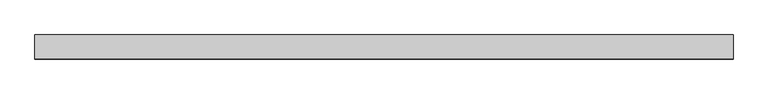
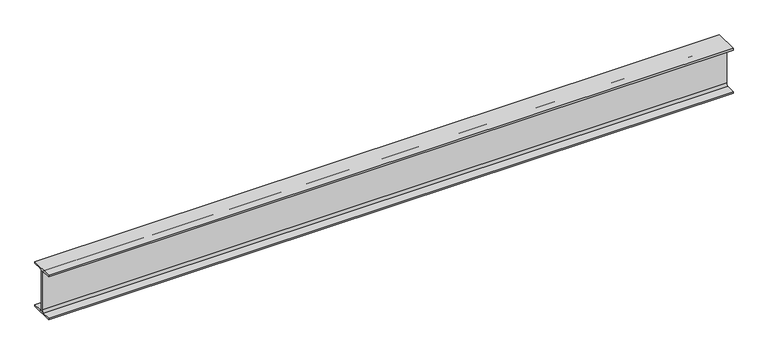
"""IFC4 building model written with IfcOpenShell, lengths in millimetres: beam geometry, 0912_Steel Framing_H-KSD3502 : H_SB_ASB_H-250x125x6x9."""

import ifcopenshell
import ifcopenshell.guid

model = None  # the IFC model being written
_history = None  # IfcOwnerHistory: only IFC2X3 demands one
_inside = {}  # id of a spatial element -> (the spatial element, [elements in it])
_under = {}  # id of a project, library or spatial element -> (it, [spatial elements below it])
_declared = {}  # id of a project -> (the project, [libraries it declares])
_typed = {}  # id of a type object -> (the type object, [elements of that type])
_made_of = {}  # id of a material, layer set ... -> (it, [elements and type objects made of it])


def new_model(schema):
    """Start an empty IFC model of exactly this schema.

    Asked for "IFC4X3", IfcOpenShell would pick the latest addendum, in which some entities
    have other attributes; the version numbers below select the first issue.
    IFC2X3 requires an IfcOwnerHistory on every rooted entity: one is made here for all.
    """
    global model, _history
    if schema == "IFC4X3":
        model = ifcopenshell.file(schema_version=(4, 3, 0, 0))
    else:
        model = ifcopenshell.file(schema=schema)
    _inside.clear()
    _under.clear()
    _declared.clear()
    _typed.clear()
    _made_of.clear()
    _history = None
    if model.schema == "IFC2X3":
        org = make("IfcOrganization", Name="unknown")
        user = make(
            "IfcPersonAndOrganization",
            ThePerson=make("IfcPerson", FamilyName="unknown"),
            TheOrganization=org,
        )
        app = make(
            "IfcApplication",
            ApplicationDeveloper=org,
            Version="unknown",
            ApplicationFullName="unknown",
            ApplicationIdentifier="unknown",
        )
        _history = make(
            "IfcOwnerHistory",
            OwningUser=user,
            OwningApplication=app,
            ChangeAction="ADDED",
            CreationDate=0,
        )
    return model


def make(cls, **values):
    """One entity of the class cls with the attributes given. An attribute that is None is left unset."""
    return model.create_entity(
        cls, **{name: value for name, value in values.items() if value is not None}
    )


def rooted(cls, **values):
    """An entity with a GlobalId (a new one), such as an element, a storey or a relation."""
    return make(cls, GlobalId=ifcopenshell.guid.new(), OwnerHistory=_history, **values)


def si_unit(unit_type, name, prefix=None):
    """IfcSIUnit, for example si_unit("LENGTHUNIT", "METRE", prefix="MILLI")."""
    return make("IfcSIUnit", UnitType=unit_type, Prefix=prefix, Name=name)


def assignment(units):
    """IfcUnitAssignment: the units of a project."""
    return None if units is None else make("IfcUnitAssignment", Units=units)


def point(xyz):
    """IfcCartesianPoint."""
    return None if xyz is None else make("IfcCartesianPoint", Coordinates=xyz)


def direction(xyz):
    """IfcDirection."""
    return None if xyz is None else make("IfcDirection", DirectionRatios=xyz)


def frame(location, z_axis=None, x_axis=None):
    """IfcAxis2Placement3D, a coordinate frame: its origin and axes. An axis left out is left unset."""
    return make(
        "IfcAxis2Placement3D",
        Location=point(location),
        Axis=direction(z_axis),
        RefDirection=direction(x_axis),
    )


def frame_2d(location, x_axis=None):
    """IfcAxis2Placement2D, a coordinate frame in the plane: its origin and x axis."""
    return make(
        "IfcAxis2Placement2D", Location=point(location), RefDirection=direction(x_axis)
    )


def origin():
    """The frame at (0, 0, 0) with its axes left unset."""
    return frame((0.0, 0.0, 0.0))


def place(relative_to, where):
    """IfcLocalPlacement: puts the frame where relative to a parent placement (None: the world)."""
    return make(
        "IfcLocalPlacement", PlacementRelTo=relative_to, RelativePlacement=where
    )


def context(
    kind, dimensions, precision=None, world=None, true_north=None, identifier=None
):
    """IfcGeometricRepresentationContext, for example the 3D "Model" context."""
    return make(
        "IfcGeometricRepresentationContext",
        ContextIdentifier=identifier,
        ContextType=kind,
        CoordinateSpaceDimension=dimensions,
        Precision=precision,
        WorldCoordinateSystem=world,
        TrueNorth=true_north,
    )


def project(units=None, contexts=None):
    """IfcProject with its units and contexts."""
    return rooted(
        "IfcProject",
        Name="project",
        RepresentationContexts=contexts,
        UnitsInContext=assignment(units),
    )


def spatial(cls, under=None, at=None, **own):
    """A site, building, storey or space (cls), placed at a placement, below another one or the project."""
    s = rooted(cls, ObjectPlacement=at, **own)
    if under is not None:
        _under.setdefault(under.id(), (under, []))[1].append(s)
    return s


def polyline(points):
    """IfcPolyline through the points."""
    return make("IfcPolyline", Points=[point(p) for p in points])


def circle_curve(where, radius):
    """IfcCircle in the frame where."""
    return make("IfcCircle", Position=where, Radius=radius)


def trimmed(basis, trim1, trim2, sense, master):
    """IfcTrimmedCurve: the piece of a basis curve between two trims."""
    return make(
        "IfcTrimmedCurve",
        BasisCurve=basis,
        Trim1=trim1,
        Trim2=trim2,
        SenseAgreement=sense,
        MasterRepresentation=master,
    )


def segment(curve, same_sense, transition):
    """IfcCompositeCurveSegment."""
    return make(
        "IfcCompositeCurveSegment",
        Transition=transition,
        SameSense=same_sense,
        ParentCurve=curve,
    )


def composite_curve(segments, self_intersect=None):
    """IfcCompositeCurve: segments joined end to end."""
    return make("IfcCompositeCurve", Segments=segments, SelfIntersect=self_intersect)


def outline(outer, holes=None, kind="AREA"):
    """IfcArbitraryClosedProfileDef: a profile drawn as a closed curve; with holes, ...WithVoids."""
    if holes is None:
        return make("IfcArbitraryClosedProfileDef", ProfileType=kind, OuterCurve=outer)
    return make(
        "IfcArbitraryProfileDefWithVoids",
        ProfileType=kind,
        OuterCurve=outer,
        InnerCurves=holes,
    )


def extrude(swept, where, along, depth):
    """IfcExtrudedAreaSolid: the profile swept, set in the frame where, extruded along a direction by depth."""
    return make(
        "IfcExtrudedAreaSolid",
        SweptArea=swept,
        Position=where,
        ExtrudedDirection=direction(along),
        Depth=depth,
    )


def shape(context_of_items, identifier, shape_type, items):
    """IfcShapeRepresentation: the items that make up one representation, for example the "Body"."""
    return make(
        "IfcShapeRepresentation",
        ContextOfItems=context_of_items,
        RepresentationIdentifier=identifier,
        RepresentationType=shape_type,
        Items=items,
    )


def source(mapping_origin, context_of_items, identifier, shape_type, items):
    """IfcRepresentationMap: a shape defined once, which mapped items show again and again."""
    return make(
        "IfcRepresentationMap",
        MappingOrigin=mapping_origin,
        MappedRepresentation=shape(context_of_items, identifier, shape_type, items),
    )


def transform(
    local_origin,
    x_axis=None,
    y_axis=None,
    z_axis=None,
    scale=None,
    scale2=None,
    scale3=None,
    uniform=True,
):
    """IfcCartesianTransformationOperator3D, or its non-uniform kind. x_axis, y_axis, z_axis: its Axis1, 2, 3."""
    if uniform:
        return make(
            "IfcCartesianTransformationOperator3D",
            Axis1=direction(x_axis),
            Axis2=direction(y_axis),
            LocalOrigin=point(local_origin),
            Scale=scale,
            Axis3=direction(z_axis),
        )
    return make(
        "IfcCartesianTransformationOperator3DnonUniform",
        Axis1=direction(x_axis),
        Axis2=direction(y_axis),
        LocalOrigin=point(local_origin),
        Scale=scale,
        Axis3=direction(z_axis),
        Scale2=scale2,
        Scale3=scale3,
    )


def mapped(mapping_source, mapping_target):
    """IfcMappedItem: shows the shape of a source again, moved by a transform."""
    return make(
        "IfcMappedItem", MappingSource=mapping_source, MappingTarget=mapping_target
    )


def made_of(thing, what):
    """Note that an element or type object is made of a material, layer set ...; save() writes the relation."""
    if what is not None:
        _made_of.setdefault(what.id(), (what, []))[1].append(thing)
    return thing


def element(
    cls,
    number,
    at=None,
    inside=None,
    cuts=None,
    type_object=None,
    material=None,
    context=None,
    identifier="Body",
    shape_type=None,
    held_by="IfcProductDefinitionShape",
    body=None,
    shapes=None,
    **own,
):
    """One element of the class cls, such as IfcWall. Its Tag is "e" and its number.

    at: its placement. inside: the storey or other place that contains it. cuts: it is an
    opening in that element (IfcRelVoidsElement). A single representation is given by context,
    identifier, shape_type and body (its items); several are given by shapes. held_by: the class
    of the entity that holds the representations. save() writes the other relations.
    """
    e = rooted(cls, Tag="e%d" % number, ObjectPlacement=at, **own)
    if body is not None:
        shapes = [shape(context, identifier, shape_type, body)]
    if shapes is not None:
        e.Representation = make(held_by, Representations=shapes)
    if inside is not None:
        _inside.setdefault(inside.id(), (inside, []))[1].append(e)
    if cuts is not None:
        rooted(
            "IfcRelVoidsElement", RelatingBuildingElement=cuts, RelatedOpeningElement=e
        )
    if type_object is not None:
        _typed.setdefault(type_object.id(), (type_object, []))[1].append(e)
    return made_of(e, material)


def aggregate(whole, parts):
    """IfcRelAggregates: a whole, such as a stair, and the parts it consists of."""
    return rooted("IfcRelAggregates", RelatingObject=whole, RelatedObjects=parts)


def save(model, path):
    """Write the relations noted so far, then the file.

    IfcRelAggregates (storeys below a building ...), IfcRelContainedInSpatialStructure (elements
    in a storey), IfcRelDefinesByType, IfcRelAssociatesMaterial and IfcRelDeclares: one each for
    every whole, place, type object, material and project.
    """
    for whole, parts in _under.values():
        aggregate(whole, parts)
    for where, things in _inside.values():
        rooted(
            "IfcRelContainedInSpatialStructure",
            RelatedElements=things,
            RelatingStructure=where,
        )
    for kind, things in _typed.values():
        rooted("IfcRelDefinesByType", RelatedObjects=things, RelatingType=kind)
    for what, things in _made_of.values():
        rooted("IfcRelAssociatesMaterial", RelatedObjects=things, RelatingMaterial=what)
    for by, libraries in _declared.values():
        rooted("IfcRelDeclares", RelatingContext=by, RelatedDefinitions=libraries)
    model.write(path)


def beam_acfca841(model_context):
    return source(origin(), model_context, "Body", "SweptSolid", [
        extrude(outline(composite_curve([segment(polyline([(62.5, -116.0), (62.5, -125.0), (-62.5, -125.0), (-62.5, -116.0), (-15.0, -116.0)]), True, "CONTINUOUS"), segment(trimmed(circle_curve(frame_2d((-15.0, -104.0)), 12.0), [point((-15.0, -116.0))], [point((-3.0, -104.0))], True, "CARTESIAN"), True, "CONTINUOUS"), segment(polyline([(-3.0, -104.0), (-3.0, 104.0)]), True, "CONTINUOUS"), segment(trimmed(circle_curve(frame_2d((-15.0, 104.0)), 12.0), [point((-3.0, 104.0))], [point((-15.0, 116.0))], True, "CARTESIAN"), True, "CONTINUOUS"), segment(polyline([(-15.0, 116.0), (-62.5, 116.0), (-62.5, 125.0), (62.5, 125.0), (62.5, 116.0), (15.0, 116.0)]), True, "CONTINUOUS"), segment(trimmed(circle_curve(frame_2d((15.0, 104.0)), 12.0), [point((15.0, 116.0))], [point((3.0, 104.0))], True, "CARTESIAN"), True, "CONTINUOUS"), segment(polyline([(3.0, 104.0), (3.0, -104.0)]), True, "CONTINUOUS"), segment(trimmed(circle_curve(frame_2d((15.0, -104.0)), 12.0), [point((3.0, -104.0))], [point((15.0, -116.0))], True, "CARTESIAN"), True, "CONTINUOUS"), segment(polyline([(15.0, -116.0), (62.5, -116.0)]), True, "CONTINUOUS")], self_intersect=False)), frame((-1718.3833333, 0.0, 0.0), z_axis=(1.0, 0.0, 0.0), x_axis=(0.0, 1.0, 0.0)), (0.0, 0.0, 1.0), 3623.1833333),
    ])


if __name__ == "__main__":
    model = new_model("IFC4")
    model_context = context("Model", 3, world=origin())
    ifc_project = project(units=[si_unit("LENGTHUNIT", "METRE", prefix="MILLI")], contexts=[model_context])
    site = spatial("IfcSite", under=ifc_project)
    building = spatial("IfcBuilding", under=site)
    placement = place(None, origin())
    beam_shape = beam_acfca841(model_context)
    element("IfcBeam", 1, ObjectType="0912_Steel Framing_H-KSD3502 : H_SB_ASB_H-250x125x6x9", at=placement, inside=building, context=model_context, shape_type="MappedRepresentation", body=[
        mapped(beam_shape, transform((0.0, 0.0, 0.0), x_axis=(1.0, 0.0, 0.0), y_axis=(0.0, 1.0, 0.0), z_axis=(0.0, 0.0, 1.0))),
    ])
    save(model, "model.ifc")

# Revit data of these elements
# Type "0912_Steel Framing_H-KSD3502 : H_SB_ASB_H-250x125x6x9"
#   H_WM Code_1 = "S01AA003-00001 | Main Steel Structure Fabrication Work | Shelter/Building | Light Steel - Standard (30KG/M>Weight) | Material: (   )"
#   H_WM Code_2 = "S03AA029-00001 | Main Steel Structure Erection Work | Shelter/Building | Light Steel (30KG/M>Weight) | Material: (   )"
#   H_WM Code_3 = "S01AA010-00001 | Main Steel Structure Fabrication Work | Shelter/Building | Steel Painting/Coating | for Non-Fireproofed Steel Surface, Surface Preparation, Primer, Second & Final Coat | Material: (   )"
#   H_Q'ty Cal Type Tag = "SB-Q2"
#   Width = 12.5 cm
#   Web Thickness = 0.6 cm
#   Web Fillet = 1.2 cm
#   Warping Constant = 42539.8 cm⁶
#   W = 0
#   Torsional Moment of Inertia = 7.8102 cm⁴
#   Section Area = 37.66 cm²
#   Plastic Modulus weak axis = 73.1 cm³
#   Plastic Modulus strong axis = 366.0 cm³
#   Perimeter = 0.97 m²/m
#   Nominal Weight = 29.60 kgf/m
#   Moment of Inertia weak axis = 294.00 cm⁴
#   Moment of Inertia strong axis = 4050.00 cm⁴
#   Height = 25.0 cm
#   Flange Thickness = 0.9 cm
#   Elastic Modulus weak axis = 47.0 cm³
#   Elastic Modulus strong axis = 324.0 cm³
#   Centroid Vertical = 12.5 cm
#   Centroid Horizontal = 6.25 cm
#   Ix = 40500000
#   Length [instance default] = 1.5240 m
#   Zx = 366000
#   b = 0.1250 m
#   h = 0.2500 m
#   r = 0.0120 m
#   s = 0.0060 m
#   t = 0.0090 m
#   A = 0.003766 m²
#   Structural Material [instance default] = Steel, 45-345
#   Assembly Code = ""
# Element 1 (IfcBeam, "0912_Steel Framing_H-KSD3502 : H_SB_ASB_H-250x125x6x9")
#   Structural Material = none
# Materials
#   "Steel, 45-345": class "Metal", colour RGB 189 187 185, transparency 0, Description = "Steel 345 MPa", Cost = 0
